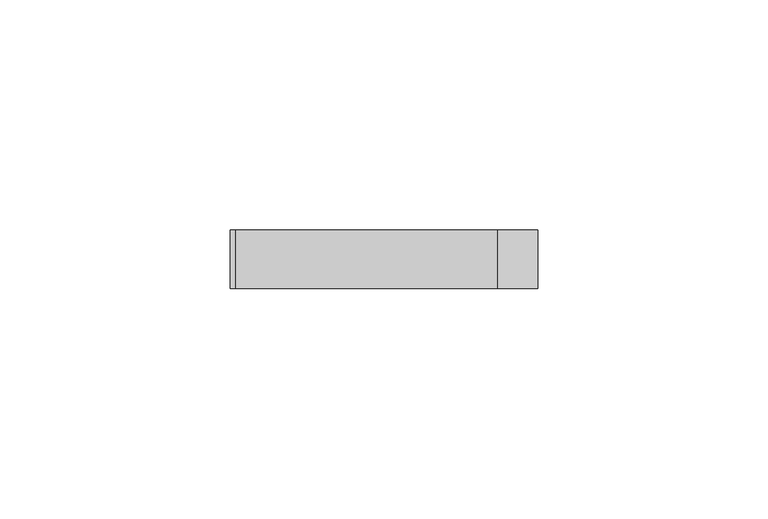
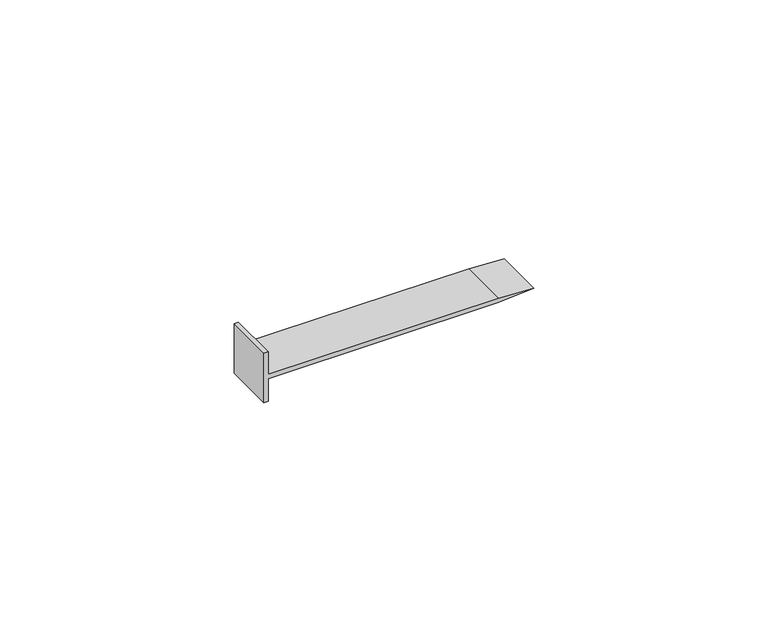
"""IFC4 building model written with IfcOpenShell, lengths in millimetres: proxy geometry, STAINLESS STEEL NAILS008 4098 : STAINLESS STEEL NAILS008 4098."""

from ifc_helpers import new_model, si_unit, frame, origin, place, context, project, spatial, polyline, outline, extrude, source, transform, mapped, element, save


def generic_models_cda5b8a7(model_context):
    return source(origin(), model_context, "Body", "SweptSolid", [
        extrude(outline(polyline([(40151.2424751, -2804.9488772), (40151.2424751, -2803.8656786), (40157.2000677, -2803.8656786), (40157.2000677, -2746.9817515), (40157.7427678, -2738.298551), (40158.2832664, -2746.9641403), (40158.2832664, -2803.8656786), (40164.240859, -2803.8656786), (40164.240859, -2804.9488772), (40151.2424751, -2804.9488772)])), frame((0.0, -1065.5906573, 0.0), z_axis=(0.0, 1.0, 0.0), x_axis=(0.0, 0.0, 1.0)), (0.0, 0.0, 1.0), 12.7),
    ])


if __name__ == "__main__":
    model = new_model("IFC4")
    model_context = context("Model", 3, world=origin())
    ifc_project = project(units=[si_unit("LENGTHUNIT", "METRE", prefix="MILLI")], contexts=[model_context])
    site = spatial("IfcSite", under=ifc_project)
    building = spatial("IfcBuilding", under=site)
    placement = place(None, origin())
    generic_models_shape = generic_models_cda5b8a7(model_context)
    element("IfcBuildingElementProxy", 1, Name="STAINLESS STEEL NAILS008 4098 : STAINLESS STEEL NAILS008 4098", ObjectType="STAINLESS STEEL NAILS008 4098 : STAINLESS STEEL NAILS008 4098", at=placement, inside=building, context=model_context, shape_type="MappedRepresentation", body=[
        mapped(generic_models_shape, transform((0.0, 0.0, 0.0), x_axis=(1.0, 0.0, 0.0), y_axis=(0.0, 1.0, 0.0), z_axis=(0.0, 0.0, 1.0))),
    ])
    save(model, "model.ifc")

# Revit data of these elements
# Type "STAINLESS STEEL NAILS008 4098 : STAINLESS STEEL NAILS008 4098"
#   NameOverride = "STAINLESS STEEL NAILS008"
# Element 1 (IfcBuildingElementProxy, "STAINLESS STEEL NAILS008 4098 : STAINLESS STEEL NAILS008 4098")
#   Materials on its faces: "1 3/4\" STAINLESS STEEL RINGSHANK 5D COMMON NAILS @ 4\" (101.6MM) O.C. FIRESTONE PROVIDED MAX., 1/2\" STAGGERED"
# Materials
#   "1 3/4\" STAINLESS STEEL RINGSHANK 5D COMMON NAILS @ 4\" (101.6MM) O.C. FIRESTONE PROVIDED MAX., 1/2\" STAGGERED": class "Unassigned", colour RGB 255 255 255, transparency 0
